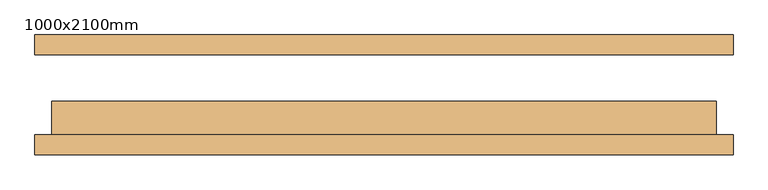
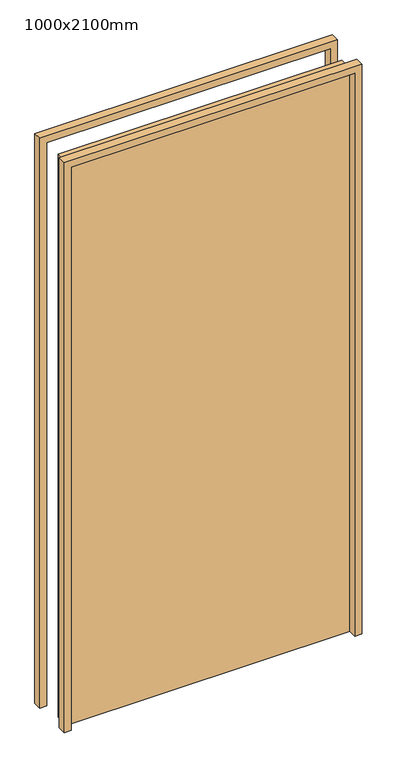
"""IFC4 building model written with IfcOpenShell, lengths in millimetres: door geometry, WWm-SingleSolid-Flush : 1000x2100mm."""

from ifc_helpers import new_model, si_unit, frame, origin, origin_with_axes, place, context, project, spatial, polyline, outline, extrude, source, transform, mapped, element, save


def door_1000x2100mm_658b1219(model_context):
    return source(origin(), model_context, "Body", "SweptSolid", [
        extrude(outline(polyline([(2125.0, -525.0), (0.0, -525.0), (0.0, -500.0), (2100.0, -500.0), (2100.0, 500.0), (0.0, 500.0), (0.0, 525.0), (2125.0, 525.0), (2125.0, -525.0)])), frame((0.0, -90.0, 0.0), z_axis=(0.0, 1.0, 0.0), x_axis=(0.0, 0.0, 1.0)), (0.0, 0.0, 1.0), 30.0),
        extrude(outline(polyline([(2125.0, 525.0), (2125.0, -525.0), (0.0, -525.0), (0.0, -500.0), (2100.0, -500.0), (2100.0, 500.0), (0.0, 500.0), (0.0, 525.0), (2125.0, 525.0)])), frame((0.0, 60.0, 0.0), z_axis=(0.0, 1.0, 0.0), x_axis=(0.0, 0.0, 1.0)), (0.0, 0.0, 1.0), 30.0),
        extrude(outline(polyline([(500.0, -10.0), (500.0, -60.0), (-500.0, -60.0), (-500.0, -10.0), (500.0, -10.0)])), origin_with_axes(), (0.0, 0.0, 1.0), 2100.0),
    ])


if __name__ == "__main__":
    model = new_model("IFC4")
    model_context = context("Model", 3, world=origin())
    ifc_project = project(units=[si_unit("LENGTHUNIT", "METRE", prefix="MILLI")], contexts=[model_context])
    site = spatial("IfcSite", under=ifc_project)
    building = spatial("IfcBuilding", under=site)
    placement = place(None, origin())
    door_1000x2100mm_shape = door_1000x2100mm_658b1219(model_context)
    element("IfcDoor", 1, ObjectType="WWm-SingleSolid-Flush : 1000x2100mm", at=placement, inside=building, context=model_context, shape_type="MappedRepresentation", body=[
        mapped(door_1000x2100mm_shape, transform((0.0, 0.0, 0.0), x_axis=(1.0, 0.0, 0.0), y_axis=(0.0, 1.0, 0.0), z_axis=(0.0, 0.0, 1.0))),
    ])
    save(model, "model.ifc")

# Revit data of these elements
# Type "WWm-SingleSolid-Flush : 1000x2100mm"
#   Type Mark = "EX1-51"
#   Construction Type Id = "MDOOR"
#   Assembly Code = "C1020"
#   Analytic Construction = "Metal"
#   Thickness = 50 mm
#   Thermal Resistance (R) = 0.270117 (m²·K)/W
#   Heat Transfer Coefficient (U) = 3.7021 W/(m²·K)
#   Height = 2100 mm
#   Trim Projection Ext = 30 mm
#   Trim Projection Int = 30 mm
#   Trim Width = 25 mm
#   Width = 1000 mm
#   Not 90 Degree [instance default] = no
#   90 Degree [instance default] = yes
#   Door Material = WW-EC-RGB-White
#   Frame Material = WW-EC-RGB-White
#   Visual Light Transmittance = 0
#   Solar Heat Gain Coefficient = 0
#   Function = (empty or 0)
#   Wall Closure = (empty or 0)
# Element 1 (IfcDoor, "WWm-SingleSolid-Flush : 1000x2100mm")
#   Materials on its faces: "WW-EC-RGB-White"
# Materials
#   "WW-EC-RGB-White": class "Generic", colour RGB 255 255 255, transparency 0, Comments = "If region requests off-white, swith asset color to RGB 231-228-220", Description = "Generic Color", Cost = 0
